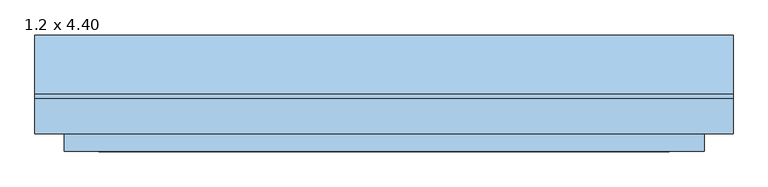
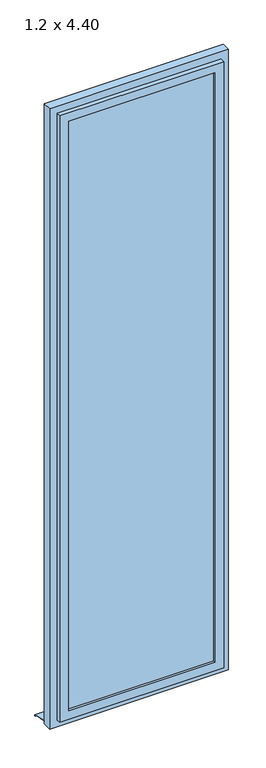
"""IFC4 building model written with IfcOpenShell, lengths in millimetres: window geometry, Fenstertür 1-flg : 1.2 x 4.40."""

from ifc_helpers import new_model, si_unit, frame, origin, place, context, project, spatial, polyline, outline, extrude, faceted_brep, source, transform, mapped, element, save


def window_1_2_x_4_40_3302ac3b(model_context):
    return source(origin(), model_context, "Body", "SolidModel", [
        extrude(outline(polyline([(4400.0, 600.0), (4400.0, -600.0), (0.0, -600.0), (0.0, 600.0), (4400.0, 600.0)]), holes=[polyline([(4320.0, 520.0), (80.0, 520.0), (80.0, -520.0), (4320.0, -520.0), (4320.0, 520.0)])]), frame((0.0, 35.0, 0.0), z_axis=(0.0, 1.0, 0.0), x_axis=(0.0, 0.0, 1.0)), (0.0, 0.0, 1.0), 60.0),
        faceted_brep([(550.0, 35.0, 4350.0), (550.0, 5.0, 4350.0), (550.0, 5.0, 50.0), (550.0, 35.0, 50.0), (-550.0, 5.0, 4350.0), (-550.0, 5.0, 50.0), (490.0, 5.0, 110.0), (-490.0, 5.0, 110.0), (-490.0, 5.0, 4290.0), (490.0, 5.0, 4290.0), (-550.0, 35.0, 50.0), (-550.0, 35.0, 4350.0), (520.0, 35.0, 4320.0), (-520.0, 35.0, 4320.0), (-520.0, 35.0, 80.0), (520.0, 35.0, 80.0), (520.0, 65.0, 4320.0), (520.0, 65.0, 80.0), (-520.0, 65.0, 80.0), (-520.0, 65.0, 4320.0), (490.0, 65.0, 4290.0), (-490.0, 65.0, 4290.0), (-490.0, 65.0, 110.0), (490.0, 65.0, 110.0)], [[[0, 1, 2, 3]], [[1, 4, 5, 2], [6, 7, 8, 9]], [[3, 2, 5, 10]], [[3, 10, 11, 0], [12, 13, 14, 15]], [[16, 12, 15, 17]], [[17, 15, 14, 18]], [[17, 18, 19, 16], [20, 21, 22, 23]], [[9, 20, 23, 6]], [[6, 23, 22, 7]], [[10, 5, 4, 11]], [[18, 14, 13, 19]], [[7, 22, 21, 8]], [[11, 4, 1, 0]], [[19, 13, 12, 16]], [[8, 21, 20, 9]]]),
        extrude(outline(polyline([(105.0221543, 20.0), (205.0, 0.0), (205.0, -10.0), (203.0, -10.0), (203.0, -1.6395366), (104.8240723, 18.0), (95.0, 18.0), (95.0, 20.0), (105.0221543, 20.0)])), frame((-600.0, 0.0, 0.0), z_axis=(1.0, 0.0, 0.0), x_axis=(0.0, 1.0, 0.0)), (0.0, 0.0, 1.0), 1200.0),
        extrude(outline(polyline([(490.0, 20.0), (-490.0, 20.0), (-490.0, 50.0), (490.0, 50.0), (490.0, 20.0)])), frame((0.0, 0.0, 110.0), z_axis=(0.0, 0.0, 1.0), x_axis=(1.0, 0.0, 0.0)), (0.0, 0.0, 1.0), 4180.0),
    ])


if __name__ == "__main__":
    model = new_model("IFC4")
    model_context = context("Model", 3, world=origin())
    ifc_project = project(units=[si_unit("LENGTHUNIT", "METRE", prefix="MILLI")], contexts=[model_context])
    site = spatial("IfcSite", under=ifc_project)
    building = spatial("IfcBuilding", under=site)
    placement = place(None, origin())
    window_1_2_x_4_40_shape = window_1_2_x_4_40_3302ac3b(model_context)
    element("IfcWindow", 1, ObjectType="Fenstertür 1-flg : 1.2 x 4.40", at=placement, inside=building, context=model_context, shape_type="MappedRepresentation", body=[
        mapped(window_1_2_x_4_40_shape, transform((0.0, 0.0, 0.0), x_axis=(1.0, 0.0, 0.0), y_axis=(0.0, 1.0, 0.0), z_axis=(0.0, 0.0, 1.0))),
    ])
    save(model, "model.ifc")

# Revit data of these elements
# Type "Fenstertür 1-flg : 1.2 x 4.40"
#   Type Mark = "56"
#   Operation = "SinglePanel"
#   Construction Type Id = "GSP4R"
#   Keynote = "16.05.01"
#   Analytic Construction = "1/8 Zoll Pilkington-Verglasung einfach"
#   Visual Light Transmittance = 0.9
#   Thermal Resistance (R) = 0.1491 (m²·K)/W
#   Solar Heat Gain Coefficient = 0.86
#   Rough Width = 1.200 m
#   Rough Height = 4.400 m
#   Heat Transfer Coefficient (U) = 6.7069 W/(m²·K)
#   Rahmentiefe = 0.060 m
#   Rahmenhöhe - unten = 0.080 m
#   Rahmenhöhe - oben = 0.080 m
#   Rahmenbreite = 0.080 m
#   Height = 4.400 m
#   Tiefe Flügel = 0.060 m
#   Flügelbreite = 0.060 m
#   Einbautiefe (von außen) [instance default] = 0.080 m
#   Width = 1.200 m
#   Kippflügel [instance default] = yes
#   Drehflügel im Grundriss darstellen [instance default] = yes
#   Drehflügel 1 [instance default] = yes
#   Rahmen 1 [instance default] = none
#   Glas [instance default] = none
#   Flügel [instance default] = none
#   Fensterbank Außenseite [instance default] = none
#   Wall Closure = (empty or 0)
# Element 1 (IfcWindow, "Fenstertür 1-flg : 1.2 x 4.40")
#   Materials on its faces: "Kunststoff - Weiß", "Glas"
# Materials
#   "Kunststoff - Weiß": class "Kunststoff", colour RGB 249 249 249, transparency 0, Cost = 0
#   "Glas": class "Glas", colour RGB 0 0 255, transparency 0.75, Comments = "Render-Darstellung nicht aktualisiert ", Cost = 0
